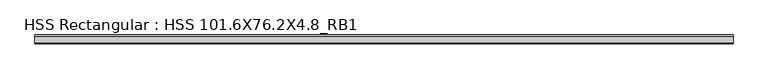
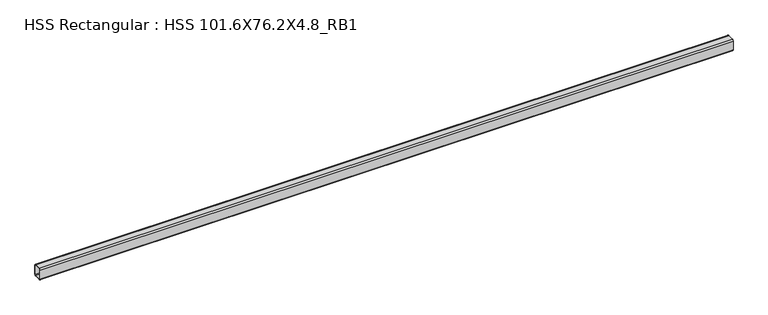
"""IFC4 building model written with IfcOpenShell, lengths in millimetres: beam geometry, HSS Rectangular : HSS 101.6X76.2X4.8_RB1."""

from ifc_helpers import new_model, si_unit, point, frame, frame_2d, origin, place, context, project, spatial, polyline, circle_curve, trimmed, segment, composite_curve, outline, extrude, source, transform, mapped, element, save


def hss_rectangular_hss_101_6x76_2x4_8_rb1_73850518(model_context):
    return source(origin(), model_context, "Body", "SweptSolid", [
        extrude(outline(composite_curve([segment(polyline([(38.1, 41.275), (38.1, -41.275)]), True, "CONTINUOUS"), segment(trimmed(circle_curve(frame_2d((28.575, -41.275)), 9.525), [point((38.1, -41.275))], [point((28.575, -50.8))], False, "CARTESIAN"), True, "CONTINUOUS"), segment(polyline([(28.575, -50.8), (-28.575, -50.8)]), True, "CONTINUOUS"), segment(trimmed(circle_curve(frame_2d((-28.575, -41.275)), 9.525), [point((-28.575, -50.8))], [point((-38.1, -41.275))], False, "CARTESIAN"), True, "CONTINUOUS"), segment(polyline([(-38.1, -41.275), (-38.1, 41.275)]), True, "CONTINUOUS"), segment(trimmed(circle_curve(frame_2d((-28.575, 41.275)), 9.525), [point((-38.1, 41.275))], [point((-28.575, 50.8))], False, "CARTESIAN"), True, "CONTINUOUS"), segment(polyline([(-28.575, 50.8), (28.575, 50.8)]), True, "CONTINUOUS"), segment(trimmed(circle_curve(frame_2d((28.575, 41.275)), 9.525), [point((28.575, 50.8))], [point((38.1, 41.275))], False, "CARTESIAN"), True, "CONTINUOUS")], self_intersect=False), holes=[composite_curve([segment(trimmed(circle_curve(frame_2d((-28.575, 41.275)), 4.7625), [point((-28.575, 46.0375))], [point((-33.3375, 41.275))], True, "CARTESIAN"), True, "CONTINUOUS"), segment(polyline([(-33.3375, 41.275), (-33.3375, -41.275)]), True, "CONTINUOUS"), segment(trimmed(circle_curve(frame_2d((-28.575, -41.275)), 4.7625), [point((-33.3375, -41.275))], [point((-28.575, -46.0375))], True, "CARTESIAN"), True, "CONTINUOUS"), segment(polyline([(-28.575, -46.0375), (28.575, -46.0375)]), True, "CONTINUOUS"), segment(trimmed(circle_curve(frame_2d((28.575, -41.275)), 4.7625), [point((28.575, -46.0375))], [point((33.3375, -41.275))], True, "CARTESIAN"), True, "CONTINUOUS"), segment(polyline([(33.3375, -41.275), (33.3375, 41.275)]), True, "CONTINUOUS"), segment(trimmed(circle_curve(frame_2d((28.575, 41.275)), 4.7625), [point((33.3375, 41.275))], [point((28.575, 46.0375))], True, "CARTESIAN"), True, "CONTINUOUS"), segment(polyline([(28.575, 46.0375), (-28.575, 46.0375)]), True, "CONTINUOUS")], self_intersect=False)]), frame((-7509.4611928, 0.0, 0.0), z_axis=(1.0, 0.0, 0.0), x_axis=(0.0, 1.0, 0.0)), (0.0, 0.0, 1.0), 5996.5124815),
    ])


if __name__ == "__main__":
    model = new_model("IFC4")
    model_context = context("Model", 3, world=origin())
    ifc_project = project(units=[si_unit("LENGTHUNIT", "METRE", prefix="MILLI")], contexts=[model_context])
    site = spatial("IfcSite", under=ifc_project)
    building = spatial("IfcBuilding", under=site)
    placement = place(None, origin())
    hss_rectangular_hss_101_6x76_2x4_8_rb1_shape = hss_rectangular_hss_101_6x76_2x4_8_rb1_73850518(model_context)
    element("IfcBeam", 1, ObjectType="HSS Rectangular : HSS 101.6X76.2X4.8_RB1", at=placement, inside=building, context=model_context, shape_type="MappedRepresentation", body=[
        mapped(hss_rectangular_hss_101_6x76_2x4_8_rb1_shape, transform((0.0, 0.0, 0.0), x_axis=(1.0, 0.0, 0.0), y_axis=(0.0, 1.0, 0.0), z_axis=(0.0, 0.0, 1.0))),
    ])
    save(model, "model.ifc")

# Revit data of these elements
# Type "HSS Rectangular : HSS 101.6X76.2X4.8_RB1"
#   Section Name Key = "HSS 4X3X3/16"
#   Assembly Code = "B10"
#   Width = 7.62 cm
#   Wall Nominal Thickness = 0.4763 cm
#   Wall Design Thickness = 0.442 cm
#   Torsional Moment of Inertia = 260.561 cm⁴
#   Torsional Modulus = 61.2876 cm³
#   Section Area = 14.4516 cm²
#   Plastic Modulus weak axis = 40.3122 cm³
#   Plastic Modulus strong axis = 49.1612 cm³
#   Perimeter = 0.881482 m²/m
#   Outer Fillet = 0.9525 cm
#   Nominal Weight = 12.1285 kgf/m
#   Moment of Inertia weak axis = 131.529 cm⁴
#   Moment of Inertia strong axis = 205.202 cm⁴
#   Inner Fillet = 0.4763 cm
#   Height = 10.16 cm
#   Elastic Modulus weak axis = 34.4128 cm³
#   Elastic Modulus strong axis = 40.476 cm³
#   Centroid Vertical = 5.08 cm
#   Centroid Horizontal = 3.81 cm
#   Length [instance default] = 1524 mm
#   Structural Material [instance default] = Steel ASTM A500, Grade B, Rectangular and Square
#   Principal Axes Angle = 0
# Element 1 (IfcBeam, "HSS Rectangular : HSS 101.6X76.2X4.8_RB1")
#   Structural Material = Steel ASTM A992
#   Materials on its faces: "Steel ASTM A992"
# Materials
#   "Steel ASTM A500, Grade B, Rectangular and Square": class "Metal", colour RGB 199 199 199, transparency 0, Description = "Carbon steel", Cost = 0
#   "Steel ASTM A992": class "Metal", colour RGB 199 199 199, transparency 0, Description = "Structural steel 50ksi", Cost = 0
